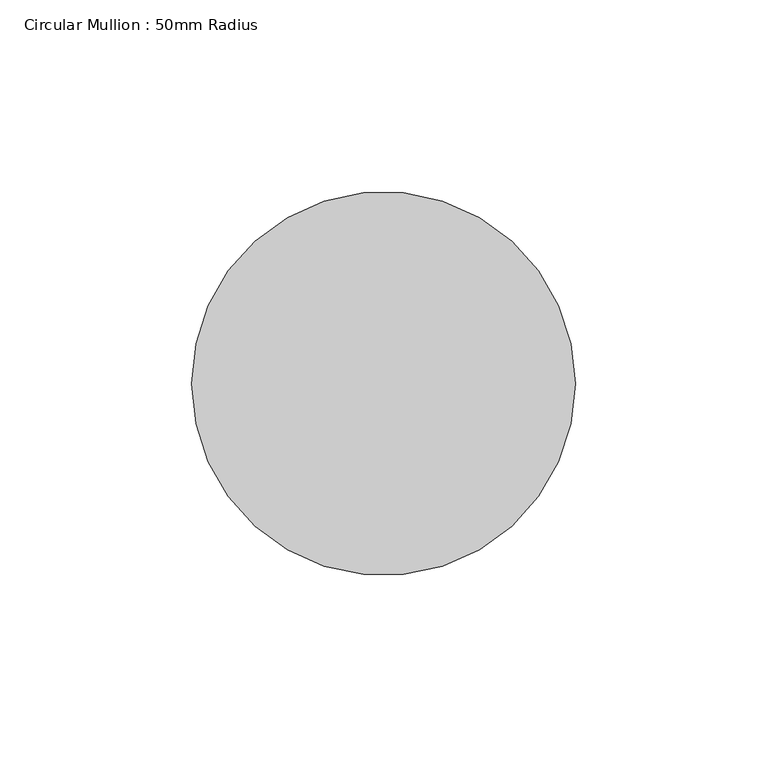
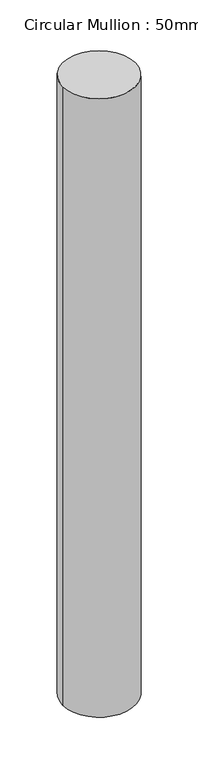
"""IFC4 building model written with IfcOpenShell, lengths in millimetres: member geometry, Circular Mullion : 50mm Radius."""

from ifc_helpers import new_model, si_unit, point, frame, origin, origin_2d, place, context, project, spatial, circle_curve, trimmed, segment, composite_curve, outline, extrude, source, transform, mapped, element, save


def circular_mullion_50mm_radius_bdae6fc5(model_context):
    return source(origin(), model_context, "Body", "SweptSolid", [
        extrude(outline(composite_curve([segment(trimmed(circle_curve(origin_2d(), 50.0), [point((50.0, 0.0))], [point((-50.0, 0.0))], False, "CARTESIAN"), True, "CONTINUOUS"), segment(trimmed(circle_curve(origin_2d(), 50.0), [point((-50.0, 0.0))], [point((50.0, 0.0))], False, "CARTESIAN"), True, "CONTINUOUS")], self_intersect=False)), frame((0.0, 0.0, -900.1800264), z_axis=(0.0, 0.0, 1.0), x_axis=(1.0, 0.0, 0.0)), (0.0, 0.0, 1.0), 900.1800264),
    ])


if __name__ == "__main__":
    model = new_model("IFC4")
    model_context = context("Model", 3, world=origin())
    ifc_project = project(units=[si_unit("LENGTHUNIT", "METRE", prefix="MILLI")], contexts=[model_context])
    site = spatial("IfcSite", under=ifc_project)
    building = spatial("IfcBuilding", under=site)
    placement = place(None, origin())
    circular_mullion_50mm_radius_shape = circular_mullion_50mm_radius_bdae6fc5(model_context)
    element("IfcMember", 1, ObjectType="Circular Mullion : 50mm Radius", at=placement, inside=building, context=model_context, shape_type="MappedRepresentation", body=[
        mapped(circular_mullion_50mm_radius_shape, transform((0.0, 0.0, 0.0), x_axis=(1.0, 0.0, 0.0), y_axis=(0.0, 1.0, 0.0), z_axis=(0.0, 0.0, 1.0))),
    ])
    save(model, "model.ifc")

# Revit data of these elements
# Type "Circular Mullion : 50mm Radius"
#   built-in parameter 1007350 = 0.164042 (stored number, unit not read)
# Element 1 (IfcMember, "Circular Mullion : 50mm Radius")
#   Materials on its faces: "Aluminium"
# Materials
#   "Aluminium": class "Metal", colour RGB 247 247 247, transparency 0, Description = "Aluminium 6061", Cost = 0
